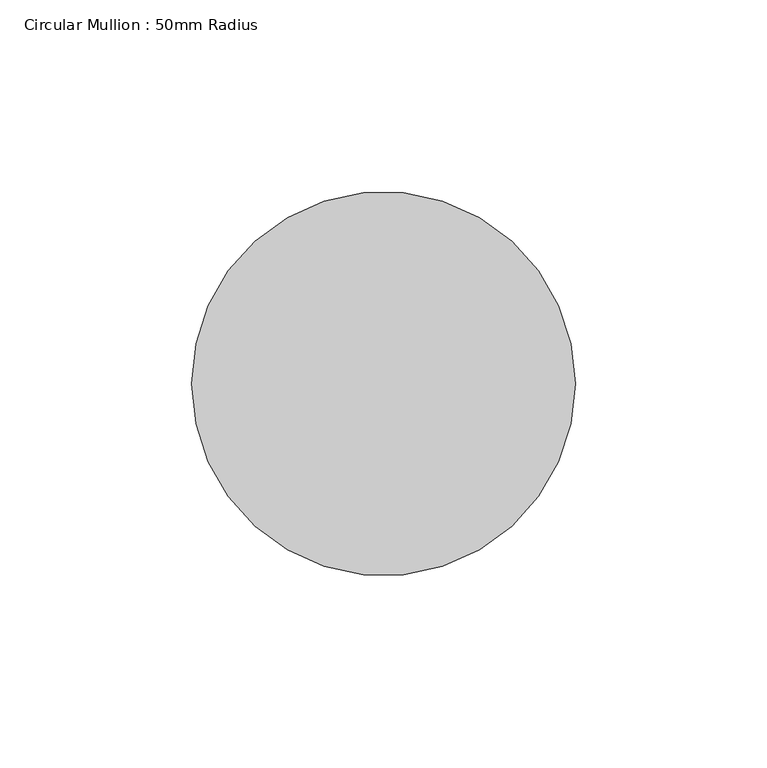
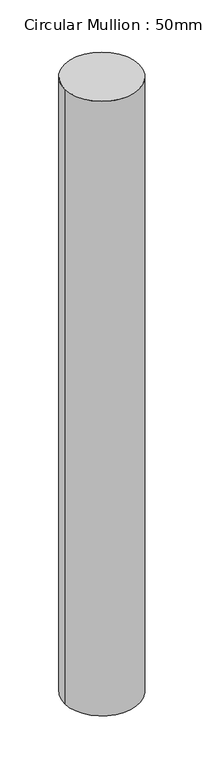
"""IFC4 building model written with IfcOpenShell, lengths in millimetres: member geometry, Circular Mullion : 50mm Radius."""

from ifc_helpers import new_model, si_unit, point, frame, origin, origin_2d, place, context, project, spatial, circle_curve, trimmed, segment, composite_curve, outline, extrude, source, transform, mapped, element, save


def circular_mullion_50mm_radius_9009f2b1(model_context):
    return source(origin(), model_context, "Body", "SweptSolid", [
        extrude(outline(composite_curve([segment(trimmed(circle_curve(origin_2d(), 50.0), [point((50.0, 0.0))], [point((-50.0, 0.0))], False, "CARTESIAN"), True, "CONTINUOUS"), segment(trimmed(circle_curve(origin_2d(), 50.0), [point((-50.0, 0.0))], [point((50.0, 0.0))], False, "CARTESIAN"), True, "CONTINUOUS")], self_intersect=False)), frame((0.0, 0.0, -872.3235529), z_axis=(0.0, 0.0, 1.0), x_axis=(1.0, 0.0, 0.0)), (0.0, 0.0, 1.0), 872.3235529),
    ])


if __name__ == "__main__":
    model = new_model("IFC4")
    model_context = context("Model", 3, world=origin())
    ifc_project = project(units=[si_unit("LENGTHUNIT", "METRE", prefix="MILLI")], contexts=[model_context])
    site = spatial("IfcSite", under=ifc_project)
    building = spatial("IfcBuilding", under=site)
    placement = place(None, origin())
    circular_mullion_50mm_radius_shape = circular_mullion_50mm_radius_9009f2b1(model_context)
    element("IfcMember", 1, ObjectType="Circular Mullion : 50mm Radius", at=placement, inside=building, context=model_context, shape_type="MappedRepresentation", body=[
        mapped(circular_mullion_50mm_radius_shape, transform((0.0, 0.0, 0.0), x_axis=(1.0, 0.0, 0.0), y_axis=(0.0, 1.0, 0.0), z_axis=(0.0, 0.0, 1.0))),
    ])
    save(model, "model.ifc")

# Revit data of these elements
# Type "Circular Mullion : 50mm Radius"
#   built-in parameter 1007350 = 0.164042 (stored number, unit not read)
# Element 1 (IfcMember, "Circular Mullion : 50mm Radius")
#   Materials on its faces: "Aluminium"
# Materials
#   "Aluminium": class "Metal", colour RGB 247 247 247, transparency 0, Description = "Aluminium 6061", Cost = 0
